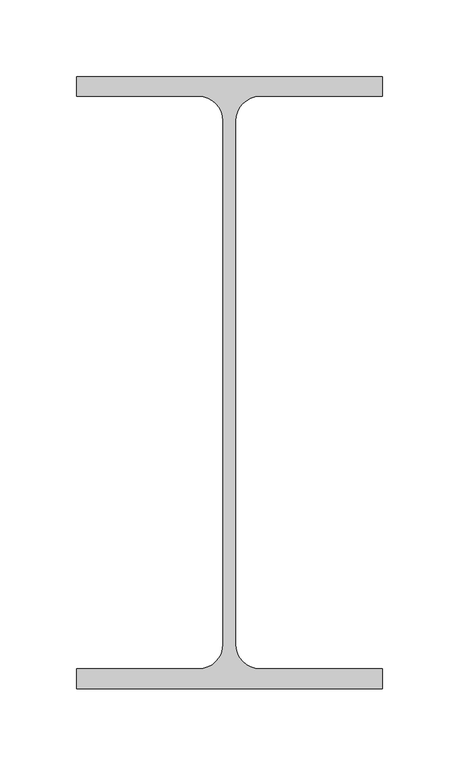
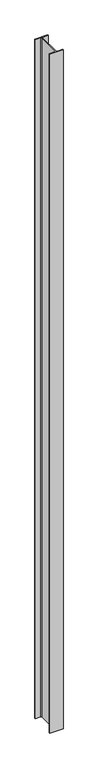
"""IFC4 building model written with IfcOpenShell, lengths in millimetres: column geometry, 0912_Steel Column_H_KSD3502 : H_SC_ASC_H-400x200x8x13."""

from ifc_helpers import new_model, si_unit, point, frame, frame_2d, origin, place, context, project, spatial, polyline, circle_curve, trimmed, segment, composite_curve, outline, extrude, source, transform, mapped, element, save


def column_1d3624df(model_context):
    return source(origin(), model_context, "Body", "SweptSolid", [
        extrude(outline(composite_curve([segment(polyline([(100.0, 200.0), (100.0, 187.0), (20.0, 187.0)]), True, "CONTINUOUS"), segment(trimmed(circle_curve(frame_2d((20.0, 171.0)), 16.0), [point((20.0, 187.0))], [point((4.0, 171.0))], True, "CARTESIAN"), True, "CONTINUOUS"), segment(polyline([(4.0, 171.0), (4.0, -171.0)]), True, "CONTINUOUS"), segment(trimmed(circle_curve(frame_2d((20.0, -171.0)), 16.0), [point((4.0, -171.0))], [point((20.0, -187.0))], True, "CARTESIAN"), True, "CONTINUOUS"), segment(polyline([(20.0, -187.0), (100.0, -187.0), (100.0, -200.0), (-100.0, -200.0), (-100.0, -187.0), (-20.0, -187.0)]), True, "CONTINUOUS"), segment(trimmed(circle_curve(frame_2d((-20.0, -171.0)), 16.0), [point((-20.0, -187.0))], [point((-4.0, -171.0))], True, "CARTESIAN"), True, "CONTINUOUS"), segment(polyline([(-4.0, -171.0), (-4.0, 171.0)]), True, "CONTINUOUS"), segment(trimmed(circle_curve(frame_2d((-20.0, 171.0)), 16.0), [point((-4.0, 171.0))], [point((-20.0, 187.0))], True, "CARTESIAN"), True, "CONTINUOUS"), segment(polyline([(-20.0, 187.0), (-100.0, 187.0), (-100.0, 200.0), (100.0, 200.0)]), True, "CONTINUOUS")], self_intersect=False)), frame((0.0, 0.0, 6949.9720055), z_axis=(0.0, 0.0, 1.0), x_axis=(1.0, 0.0, 0.0)), (0.0, 0.0, 1.0), 11000.0),
    ])


if __name__ == "__main__":
    model = new_model("IFC4")
    model_context = context("Model", 3, world=origin())
    ifc_project = project(units=[si_unit("LENGTHUNIT", "METRE", prefix="MILLI")], contexts=[model_context])
    site = spatial("IfcSite", under=ifc_project)
    building = spatial("IfcBuilding", under=site)
    placement = place(None, origin())
    column_shape = column_1d3624df(model_context)
    element("IfcColumn", 1, ObjectType="0912_Steel Column_H_KSD3502 : H_SC_ASC_H-400x200x8x13", at=placement, inside=building, context=model_context, shape_type="MappedRepresentation", body=[
        mapped(column_shape, transform((0.0, 0.0, 0.0), x_axis=(1.0, 0.0, 0.0), y_axis=(0.0, 1.0, 0.0), z_axis=(0.0, 0.0, 1.0))),
    ])
    save(model, "model.ifc")

# Revit data of these elements
# Type "0912_Steel Column_H_KSD3502 : H_SC_ASC_H-400x200x8x13"
#   H_WM Code_1 = "S01AA002-00001 | Main Steel Structure Fabrication Work | Shelter/Building | Medium Steel - Standard (90KG/M>Weight≥30KG/M) | Material: (   )"
#   H_WM Code_2 = "S03AA028-00001 | Main Steel Structure Erection Work | Shelter/Building | Medium Steel (90KG/M>Weight≥30KG/M) | Material: (   )"
#   H_WM Code_3 = "S01AA010-00001 | Main Steel Structure Fabrication Work | Shelter/Building | Steel Painting/Coating | for Non-Fireproofed Steel Surface, Surface Preparation, Primer, Second & Final Coat | Material: (   )"
#   H_Q'ty Cal Type Tag = "SC-Q2"
#   Width = 20.0 cm
#   Web Thickness = 0.8 cm
#   Web Fillet = 1.6 cm
#   Warping Constant = 648999.0 cm⁶
#   Torsional Moment of Inertia = 35.8981 cm⁴
#   Section Area = 84.12 cm²
#   Plastic Modulus weak axis = 268.0 cm³
#   Plastic Modulus strong axis = 1330.0 cm³
#   Perimeter = 1.56 m²/m
#   Nominal Weight = 66.00 kgf/m
#   Moment of Inertia weak axis = 1740.00 cm⁴
#   Moment of Inertia strong axis = 23700.00 cm⁴
#   Height = 40.0 cm
#   Flange Thickness = 1.3 cm
#   Elastic Modulus weak axis = 174.0 cm³
#   Elastic Modulus strong axis = 1190.0 cm³
#   Centroid Vertical = 20.0 cm
#   Centroid Horizontal = 10.0 cm
#   Structural Material [instance default] = Steel, 45-345
#   Section Name Key = ""
#   Bolt Spacing = 0
#   Assembly Code = ""
# Element 1 (IfcColumn, "0912_Steel Column_H_KSD3502 : H_SC_ASC_H-400x200x8x13")
#   Structural Material = none
# Materials
#   "Steel, 45-345": class "Metal", colour RGB 189 187 185, transparency 0, Description = "Steel 345 MPa", Cost = 0
